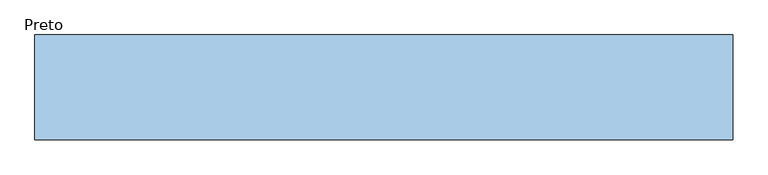
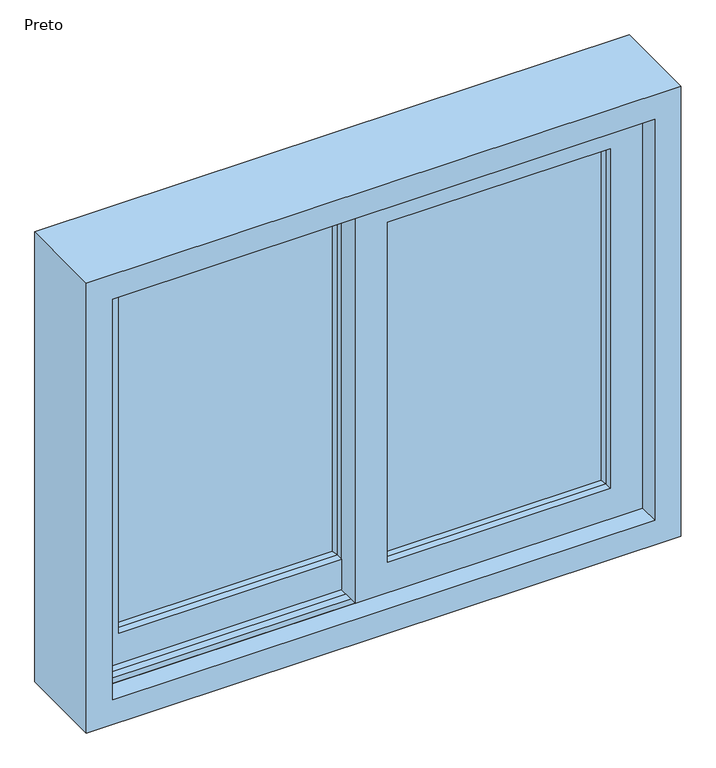
"""IFC4 building model written with IfcOpenShell, lengths in millimetres: window geometry, Blks_Cons Weiku_Janela de Correr 02 Folhas : Preto."""

import ifcopenshell
import ifcopenshell.guid

model = None  # the IFC model being written
_history = None  # IfcOwnerHistory: only IFC2X3 demands one
_inside = {}  # id of a spatial element -> (the spatial element, [elements in it])
_under = {}  # id of a project, library or spatial element -> (it, [spatial elements below it])
_declared = {}  # id of a project -> (the project, [libraries it declares])
_typed = {}  # id of a type object -> (the type object, [elements of that type])
_made_of = {}  # id of a material, layer set ... -> (it, [elements and type objects made of it])


def new_model(schema):
    """Start an empty IFC model of exactly this schema.

    Asked for "IFC4X3", IfcOpenShell would pick the latest addendum, in which some entities
    have other attributes; the version numbers below select the first issue.
    IFC2X3 requires an IfcOwnerHistory on every rooted entity: one is made here for all.
    """
    global model, _history
    if schema == "IFC4X3":
        model = ifcopenshell.file(schema_version=(4, 3, 0, 0))
    else:
        model = ifcopenshell.file(schema=schema)
    _inside.clear()
    _under.clear()
    _declared.clear()
    _typed.clear()
    _made_of.clear()
    _history = None
    if model.schema == "IFC2X3":
        org = make("IfcOrganization", Name="unknown")
        user = make(
            "IfcPersonAndOrganization",
            ThePerson=make("IfcPerson", FamilyName="unknown"),
            TheOrganization=org,
        )
        app = make(
            "IfcApplication",
            ApplicationDeveloper=org,
            Version="unknown",
            ApplicationFullName="unknown",
            ApplicationIdentifier="unknown",
        )
        _history = make(
            "IfcOwnerHistory",
            OwningUser=user,
            OwningApplication=app,
            ChangeAction="ADDED",
            CreationDate=0,
        )
    return model


def make(cls, **values):
    """One entity of the class cls with the attributes given. An attribute that is None is left unset."""
    return model.create_entity(
        cls, **{name: value for name, value in values.items() if value is not None}
    )


def rooted(cls, **values):
    """An entity with a GlobalId (a new one), such as an element, a storey or a relation."""
    return make(cls, GlobalId=ifcopenshell.guid.new(), OwnerHistory=_history, **values)


def si_unit(unit_type, name, prefix=None):
    """IfcSIUnit, for example si_unit("LENGTHUNIT", "METRE", prefix="MILLI")."""
    return make("IfcSIUnit", UnitType=unit_type, Prefix=prefix, Name=name)


def assignment(units):
    """IfcUnitAssignment: the units of a project."""
    return None if units is None else make("IfcUnitAssignment", Units=units)


def point(xyz):
    """IfcCartesianPoint."""
    return None if xyz is None else make("IfcCartesianPoint", Coordinates=xyz)


def direction(xyz):
    """IfcDirection."""
    return None if xyz is None else make("IfcDirection", DirectionRatios=xyz)


def frame(location, z_axis=None, x_axis=None):
    """IfcAxis2Placement3D, a coordinate frame: its origin and axes. An axis left out is left unset."""
    return make(
        "IfcAxis2Placement3D",
        Location=point(location),
        Axis=direction(z_axis),
        RefDirection=direction(x_axis),
    )


def origin():
    """The frame at (0, 0, 0) with its axes left unset."""
    return frame((0.0, 0.0, 0.0))


def place(relative_to, where):
    """IfcLocalPlacement: puts the frame where relative to a parent placement (None: the world)."""
    return make(
        "IfcLocalPlacement", PlacementRelTo=relative_to, RelativePlacement=where
    )


def context(
    kind, dimensions, precision=None, world=None, true_north=None, identifier=None
):
    """IfcGeometricRepresentationContext, for example the 3D "Model" context."""
    return make(
        "IfcGeometricRepresentationContext",
        ContextIdentifier=identifier,
        ContextType=kind,
        CoordinateSpaceDimension=dimensions,
        Precision=precision,
        WorldCoordinateSystem=world,
        TrueNorth=true_north,
    )


def project(units=None, contexts=None):
    """IfcProject with its units and contexts."""
    return rooted(
        "IfcProject",
        Name="project",
        RepresentationContexts=contexts,
        UnitsInContext=assignment(units),
    )


def spatial(cls, under=None, at=None, **own):
    """A site, building, storey or space (cls), placed at a placement, below another one or the project."""
    s = rooted(cls, ObjectPlacement=at, **own)
    if under is not None:
        _under.setdefault(under.id(), (under, []))[1].append(s)
    return s


def polyline(points):
    """IfcPolyline through the points."""
    return make("IfcPolyline", Points=[point(p) for p in points])


def outline(outer, holes=None, kind="AREA"):
    """IfcArbitraryClosedProfileDef: a profile drawn as a closed curve; with holes, ...WithVoids."""
    if holes is None:
        return make("IfcArbitraryClosedProfileDef", ProfileType=kind, OuterCurve=outer)
    return make(
        "IfcArbitraryProfileDefWithVoids",
        ProfileType=kind,
        OuterCurve=outer,
        InnerCurves=holes,
    )


def extrude(swept, where, along, depth):
    """IfcExtrudedAreaSolid: the profile swept, set in the frame where, extruded along a direction by depth."""
    return make(
        "IfcExtrudedAreaSolid",
        SweptArea=swept,
        Position=where,
        ExtrudedDirection=direction(along),
        Depth=depth,
    )


def faces_of(points, faces, orient=None, outer=None):
    """IfcFace entities. A face is a list of loops; a loop is a list of indices into points, from 0.

    orient and outer hold one flag for each loop. By default every Orientation is true, the
    first loop of a face is its IfcFaceOuterBound and the others are IfcFaceBound.
    """
    made = []
    for i, loops in enumerate(faces):
        bounds = []
        for j, loop in enumerate(loops):
            is_outer = j == 0 if outer is None else outer[i][j]
            bounds.append(
                make(
                    "IfcFaceOuterBound" if is_outer else "IfcFaceBound",
                    Bound=make("IfcPolyLoop", Polygon=[points[k] for k in loop]),
                    Orientation=True if orient is None else orient[i][j],
                )
            )
        made.append(make("IfcFace", Bounds=bounds))
    return made


def faceted_brep(points, faces, orient=None, outer=None, voids=None):
    """IfcFacetedBrep: a solid bounded by flat faces; with voids (closed shells), ...WithVoids."""
    shared = [point(p) for p in points]
    hull = make("IfcClosedShell", CfsFaces=faces_of(shared, faces, orient, outer))
    if voids is None:
        return make("IfcFacetedBrep", Outer=hull)
    return make(
        "IfcFacetedBrepWithVoids",
        Outer=hull,
        Voids=[
            make(cls, CfsFaces=faces_of(shared, fs, o, b)) for cls, fs, o, b in voids
        ],
    )


def shape(context_of_items, identifier, shape_type, items):
    """IfcShapeRepresentation: the items that make up one representation, for example the "Body"."""
    return make(
        "IfcShapeRepresentation",
        ContextOfItems=context_of_items,
        RepresentationIdentifier=identifier,
        RepresentationType=shape_type,
        Items=items,
    )


def source(mapping_origin, context_of_items, identifier, shape_type, items):
    """IfcRepresentationMap: a shape defined once, which mapped items show again and again."""
    return make(
        "IfcRepresentationMap",
        MappingOrigin=mapping_origin,
        MappedRepresentation=shape(context_of_items, identifier, shape_type, items),
    )


def transform(
    local_origin,
    x_axis=None,
    y_axis=None,
    z_axis=None,
    scale=None,
    scale2=None,
    scale3=None,
    uniform=True,
):
    """IfcCartesianTransformationOperator3D, or its non-uniform kind. x_axis, y_axis, z_axis: its Axis1, 2, 3."""
    if uniform:
        return make(
            "IfcCartesianTransformationOperator3D",
            Axis1=direction(x_axis),
            Axis2=direction(y_axis),
            LocalOrigin=point(local_origin),
            Scale=scale,
            Axis3=direction(z_axis),
        )
    return make(
        "IfcCartesianTransformationOperator3DnonUniform",
        Axis1=direction(x_axis),
        Axis2=direction(y_axis),
        LocalOrigin=point(local_origin),
        Scale=scale,
        Axis3=direction(z_axis),
        Scale2=scale2,
        Scale3=scale3,
    )


def mapped(mapping_source, mapping_target):
    """IfcMappedItem: shows the shape of a source again, moved by a transform."""
    return make(
        "IfcMappedItem", MappingSource=mapping_source, MappingTarget=mapping_target
    )


def made_of(thing, what):
    """Note that an element or type object is made of a material, layer set ...; save() writes the relation."""
    if what is not None:
        _made_of.setdefault(what.id(), (what, []))[1].append(thing)
    return thing


def element(
    cls,
    number,
    at=None,
    inside=None,
    cuts=None,
    type_object=None,
    material=None,
    context=None,
    identifier="Body",
    shape_type=None,
    held_by="IfcProductDefinitionShape",
    body=None,
    shapes=None,
    **own,
):
    """One element of the class cls, such as IfcWall. Its Tag is "e" and its number.

    at: its placement. inside: the storey or other place that contains it. cuts: it is an
    opening in that element (IfcRelVoidsElement). A single representation is given by context,
    identifier, shape_type and body (its items); several are given by shapes. held_by: the class
    of the entity that holds the representations. save() writes the other relations.
    """
    e = rooted(cls, Tag="e%d" % number, ObjectPlacement=at, **own)
    if body is not None:
        shapes = [shape(context, identifier, shape_type, body)]
    if shapes is not None:
        e.Representation = make(held_by, Representations=shapes)
    if inside is not None:
        _inside.setdefault(inside.id(), (inside, []))[1].append(e)
    if cuts is not None:
        rooted(
            "IfcRelVoidsElement", RelatingBuildingElement=cuts, RelatedOpeningElement=e
        )
    if type_object is not None:
        _typed.setdefault(type_object.id(), (type_object, []))[1].append(e)
    return made_of(e, material)


def aggregate(whole, parts):
    """IfcRelAggregates: a whole, such as a stair, and the parts it consists of."""
    return rooted("IfcRelAggregates", RelatingObject=whole, RelatedObjects=parts)


def save(model, path):
    """Write the relations noted so far, then the file.

    IfcRelAggregates (storeys below a building ...), IfcRelContainedInSpatialStructure (elements
    in a storey), IfcRelDefinesByType, IfcRelAssociatesMaterial and IfcRelDeclares: one each for
    every whole, place, type object, material and project.
    """
    for whole, parts in _under.values():
        aggregate(whole, parts)
    for where, things in _inside.values():
        rooted(
            "IfcRelContainedInSpatialStructure",
            RelatedElements=things,
            RelatingStructure=where,
        )
    for kind, things in _typed.values():
        rooted("IfcRelDefinesByType", RelatedObjects=things, RelatingType=kind)
    for what, things in _made_of.values():
        rooted("IfcRelAssociatesMaterial", RelatedObjects=things, RelatingMaterial=what)
    for by, libraries in _declared.values():
        rooted("IfcRelDeclares", RelatingContext=by, RelatedDefinitions=libraries)
    model.write(path)


def preto_fcda803b(model_context):
    return source(origin(), model_context, "Body", "SolidModel", [
        faceted_brep([(27.0, -13.0, 898.0), (27.0, -18.0, 898.0), (27.0, -18.0, 1502.0), (27.0, -13.0, 1502.0), (32.0, -18.0, 903.0), (32.0, -18.0, 1497.0), (402.0, -18.0, 1502.0), (402.0, -13.0, 1502.0), (397.0, -18.0, 1497.0), (402.0, -18.0, 898.0), (402.0, -13.0, 898.0), (397.0, -18.0, 903.0)], [[[0, 1, 2, 3]], [[4, 0, 3, 5]], [[3, 2, 6, 7]], [[5, 3, 7, 8]], [[7, 6, 9, 10]], [[8, 7, 10, 11]], [[1, 9, 6, 2], [5, 8, 11, 4]], [[10, 9, 1, 0]], [[11, 10, 0, 4]]]),
        faceted_brep([(402.0, -27.0, 898.0), (402.0, -22.0, 898.0), (402.0, -22.0, 1502.0), (402.0, -27.0, 1502.0), (27.0, -22.0, 1502.0), (27.0, -27.0, 1502.0), (27.0, -22.0, 898.0), (27.0, -27.0, 898.0), (397.0, -22.0, 1497.0), (32.0, -22.0, 1497.0), (32.0, -22.0, 903.0), (397.0, -22.0, 903.0)], [[[0, 1, 2, 3]], [[3, 2, 4, 5]], [[5, 4, 6, 7]], [[1, 6, 4, 2], [8, 9, 10, 11]], [[7, 6, 1, 0]], [[11, 0, 3, 8]], [[8, 3, 5, 9]], [[9, 5, 7, 10]], [[10, 7, 0, 11]]]),
        extrude(outline(polyline([(402.0, -22.0), (27.0, -22.0), (27.0, -18.0), (402.0, -18.0), (402.0, -22.0)])), frame((0.0, 0.0, 898.0), z_axis=(0.0, 0.0, 1.0), x_axis=(1.0, 0.0, 0.0)), (0.0, 0.0, 1.0), 604.0),
        extrude(outline(polyline([(844.0, 456.0), (1556.0, 456.0), (1556.0, -27.0), (844.0, -27.0), (844.0, 456.0)]), holes=[polyline([(1502.0, 27.0), (1502.0, 402.0), (898.0, 402.0), (898.0, 27.0), (1502.0, 27.0)])]), frame((0.0, -40.0, 0.0), z_axis=(0.0, 1.0, 0.0), x_axis=(0.0, 0.0, 1.0)), (0.0, 0.0, 1.0), 40.0),
        faceted_brep([(-402.0, 27.0, 898.0), (-402.0, 22.0, 898.0), (-402.0, 22.0, 1502.0), (-402.0, 27.0, 1502.0), (-397.0, 22.0, 903.0), (-397.0, 22.0, 1497.0), (-27.0, 22.0, 1502.0), (-27.0, 27.0, 1502.0), (-32.0, 22.0, 1497.0), (-27.0, 22.0, 898.0), (-27.0, 27.0, 898.0), (-32.0, 22.0, 903.0)], [[[0, 1, 2, 3]], [[4, 0, 3, 5]], [[3, 2, 6, 7]], [[5, 3, 7, 8]], [[7, 6, 9, 10]], [[8, 7, 10, 11]], [[1, 9, 6, 2], [5, 8, 11, 4]], [[10, 9, 1, 0]], [[11, 10, 0, 4]]]),
        faceted_brep([(-27.0, 13.0, 898.0), (-27.0, 18.0, 898.0), (-27.0, 18.0, 1502.0), (-27.0, 13.0, 1502.0), (-402.0, 18.0, 1502.0), (-402.0, 13.0, 1502.0), (-402.0, 18.0, 898.0), (-402.0, 13.0, 898.0), (-32.0, 18.0, 1497.0), (-397.0, 18.0, 1497.0), (-397.0, 18.0, 903.0), (-32.0, 18.0, 903.0)], [[[0, 1, 2, 3]], [[3, 2, 4, 5]], [[5, 4, 6, 7]], [[1, 6, 4, 2], [8, 9, 10, 11]], [[7, 6, 1, 0]], [[11, 0, 3, 8]], [[8, 3, 5, 9]], [[9, 5, 7, 10]], [[10, 7, 0, 11]]]),
        extrude(outline(polyline([(-27.0, 18.0), (-402.0, 18.0), (-402.0, 22.0), (-27.0, 22.0), (-27.0, 18.0)])), frame((0.0, 0.0, 898.0), z_axis=(0.0, 0.0, 1.0), x_axis=(1.0, 0.0, 0.0)), (0.0, 0.0, 1.0), 604.0),
        extrude(outline(polyline([(844.0, 27.0), (1556.0, 27.0), (1556.0, -456.0), (844.0, -456.0), (844.0, 27.0)]), holes=[polyline([(1502.0, -402.0), (1502.0, -27.0), (898.0, -27.0), (898.0, -402.0), (1502.0, -402.0)])]), frame((0.0, 0.0, 0.0), z_axis=(0.0, 1.0, 0.0), x_axis=(0.0, 0.0, 1.0)), (0.0, 0.0, 1.0), 40.0),
        faceted_brep([(456.0, 75.0, 844.0), (-456.0, 75.0, 844.0), (-456.0, 40.0, 844.0), (456.0, 40.0, 844.0), (-456.0, -75.0, 844.0), (456.0, -75.0, 844.0), (456.0, -40.0, 844.0), (-456.0, -40.0, 844.0), (-456.0, -13.0, 844.0), (-456.0, -27.0, 844.0), (456.0, -27.0, 844.0), (456.0, -13.0, 844.0), (-456.0, 27.0, 844.0), (-456.0, 13.0, 844.0), (456.0, 13.0, 844.0), (456.0, 27.0, 844.0), (500.0, 75.0, 800.0), (-500.0, 75.0, 800.0), (-500.0, 75.0, 1600.0), (500.0, 75.0, 1600.0), (456.0, 75.0, 1556.0), (-456.0, 75.0, 1556.0), (-456.0, 40.0, 1556.0), (-456.0, 40.0, 1566.0), (-456.0, 27.0, 1566.0), (-456.0, 27.0, 1556.0), (-456.0, 13.0, 1556.0), (-456.0, 13.0, 1566.0), (-456.0, -13.0, 1566.0), (-456.0, -13.0, 1556.0), (-456.0, -27.0, 1556.0), (-456.0, -27.0, 1566.0), (-456.0, -40.0, 1566.0), (-456.0, -40.0, 1556.0), (-456.0, -75.0, 1556.0), (-456.0, -40.0, 834.0), (-456.0, -27.0, 834.0), (-456.0, -13.0, 834.0), (-456.0, 13.0, 834.0), (-456.0, 27.0, 834.0), (-456.0, 40.0, 834.0), (456.0, 40.0, 834.0), (456.0, 27.0, 834.0), (456.0, 13.0, 834.0), (456.0, -13.0, 834.0), (456.0, -27.0, 834.0), (456.0, -40.0, 834.0), (456.0, -75.0, 1556.0), (456.0, -40.0, 1556.0), (456.0, -40.0, 1566.0), (456.0, -27.0, 1566.0), (456.0, -27.0, 1556.0), (456.0, -13.0, 1556.0), (456.0, -13.0, 1566.0), (456.0, 13.0, 1566.0), (456.0, 13.0, 1556.0), (456.0, 27.0, 1556.0), (456.0, 27.0, 1566.0), (456.0, 40.0, 1566.0), (456.0, 40.0, 1556.0), (-500.0, -75.0, 800.0), (500.0, -75.0, 800.0), (500.0, -75.0, 1600.0), (-500.0, -75.0, 1600.0)], [[[0, 1, 2, 3]], [[4, 5, 6, 7]], [[8, 9, 10, 11]], [[12, 13, 14, 15]], [[16, 17, 18, 19], [1, 0, 20, 21]], [[1, 21, 22, 23, 24, 25, 26, 27, 28, 29, 30, 31, 32, 33, 34, 4, 7, 35, 36, 9, 8, 37, 38, 13, 12, 39, 40, 2]], [[40, 41, 3, 2]], [[20, 0, 3, 41, 42, 15, 14, 43, 44, 11, 10, 45, 46, 6, 5, 47, 48, 49, 50, 51, 52, 53, 54, 55, 56, 57, 58, 59]], [[60, 61, 62, 63], [5, 4, 34, 47]], [[46, 35, 7, 6]], [[45, 10, 9, 36]], [[11, 44, 37, 8]], [[43, 14, 13, 38]], [[15, 42, 39, 12]], [[61, 16, 19, 62]], [[16, 61, 60, 17]], [[17, 60, 63, 18]], [[46, 45, 36, 35]], [[44, 43, 38, 37]], [[42, 41, 40, 39]], [[26, 25, 56, 55]], [[30, 29, 52, 51]], [[21, 20, 59, 22]], [[47, 34, 33, 48]], [[18, 63, 62, 19]], [[55, 54, 27, 26]], [[54, 53, 28, 27]], [[53, 52, 29, 28]], [[51, 50, 31, 30]], [[50, 49, 32, 31]], [[32, 49, 48, 33]], [[58, 23, 22, 59]], [[58, 57, 24, 23]], [[57, 56, 25, 24]]]),
    ])


if __name__ == "__main__":
    model = new_model("IFC4")
    model_context = context("Model", 3, world=origin())
    ifc_project = project(units=[si_unit("LENGTHUNIT", "METRE", prefix="MILLI")], contexts=[model_context])
    site = spatial("IfcSite", under=ifc_project)
    building = spatial("IfcBuilding", under=site)
    placement = place(None, origin())
    preto_shape = preto_fcda803b(model_context)
    element("IfcWindow", 1, ObjectType="Blks_Cons Weiku_Janela de Correr 02 Folhas : Preto", at=placement, inside=building, context=model_context, shape_type="MappedRepresentation", body=[
        mapped(preto_shape, transform((0.0, 0.0, 0.0), x_axis=(1.0, 0.0, 0.0), y_axis=(0.0, 1.0, 0.0), z_axis=(0.0, 0.0, 1.0))),
    ])
    save(model, "model.ifc")

# Revit data of these elements
# Type "Blks_Cons Weiku_Janela de Correr 02 Folhas : Preto"
#   Type Mark = "J26"
#   Type Comments = "Janela de Correr 02 Folhas"
#   Manufacturer = "Weiku"
#   Created By / Criado Por / Creado por = "Blocks"
#   Author URL = "https://BlocksRvt.com/"
#   Author Contact = "info@blocksrvt.com"
#   Assembly Code = "Cons"
#   c [instance default] = 250 mm
#   b [instance default] = 912 mm
#   a [instance default] = 983 mm
#   Rough Width [instance default] = 2000 mm
#   Width [instance default] = 1912 mm
#   Espessura Folha [instance default] = 40 mm
#   Rough Height [instance default] = 1000 mm
#   Height [instance default] = 912 mm
#   Abertura Janela Equerda [instance default] = 0 mm
#   Abertura Janela Direita [instance default] = 0 mm
#   Vidro = .vidro_growarq
#   Vedação = Blks - Rubber - Black
#   Janela = Blks - Plastic - Black - Glazed
#   Wall Closure = (empty or 0)
# Element 1 (IfcWindow, "Blks_Cons Weiku_Janela de Correr 02 Folhas : Preto")
#   c = 200 mm
#   b = 712 mm
#   a = 483 mm
#   Rough Width = 1000 mm
#   Width = 912 mm
#   Rough Height = 800 mm
#   Height = 712 mm
#   Materials on its faces: "Blks - Plastic - Black - Glazed", "Blks - Rubber - Black", ".vidro_growarq"
# Materials
#   ".vidro_growarq": class "Vidro", colour RGB 200 215 215, transparency 0.6, Description = "Vidroverde", Cost = 0
#   "Blks - Rubber - Black": class "Paint/Coating", colour RGB 38 38 38, transparency 0, Cost = 0
#   "Blks - Plastic - Black - Glazed": class "Plastic", colour RGB 25 25 25, transparency 0, Cost = 0
